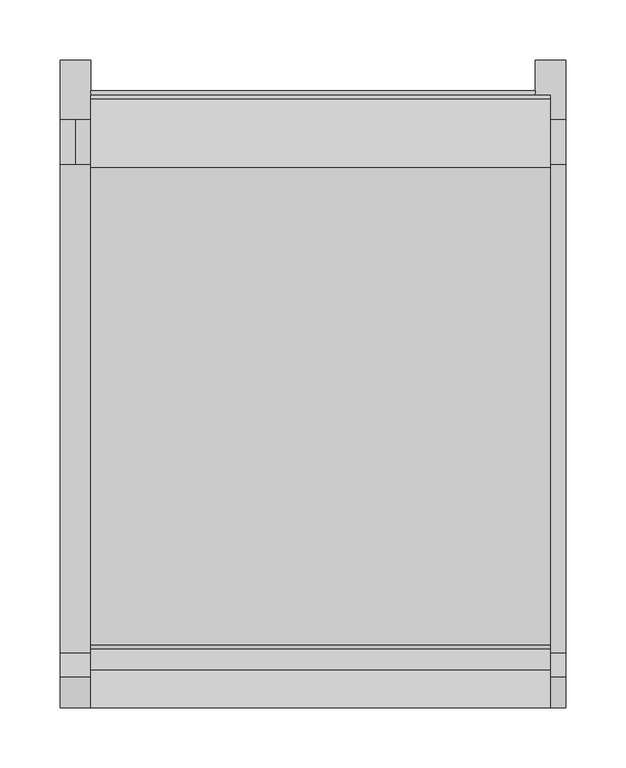
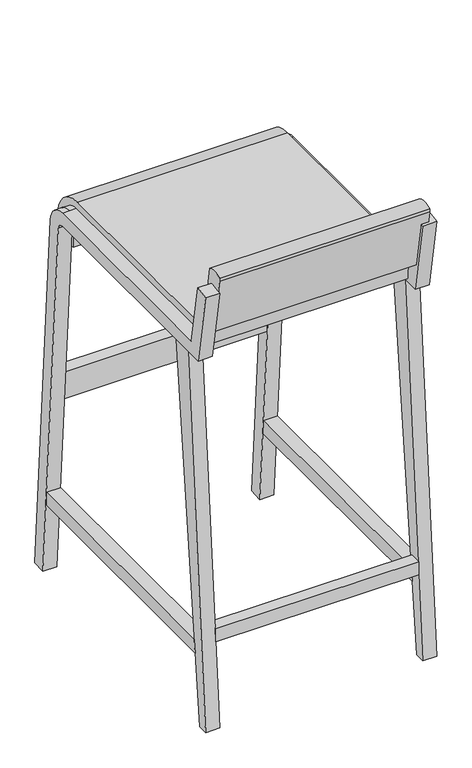
"""IFC4 building model written with IfcOpenShell, lengths in millimetres: furniture geometry, Bar_Stool_6722[1] : Bar_Stool_6722[1]."""

import ifcopenshell
import ifcopenshell.guid

model = None  # the IFC model being written
_history = None  # IfcOwnerHistory: only IFC2X3 demands one
_inside = {}  # id of a spatial element -> (the spatial element, [elements in it])
_under = {}  # id of a project, library or spatial element -> (it, [spatial elements below it])
_declared = {}  # id of a project -> (the project, [libraries it declares])
_typed = {}  # id of a type object -> (the type object, [elements of that type])
_made_of = {}  # id of a material, layer set ... -> (it, [elements and type objects made of it])


def new_model(schema):
    """Start an empty IFC model of exactly this schema.

    Asked for "IFC4X3", IfcOpenShell would pick the latest addendum, in which some entities
    have other attributes; the version numbers below select the first issue.
    IFC2X3 requires an IfcOwnerHistory on every rooted entity: one is made here for all.
    """
    global model, _history
    if schema == "IFC4X3":
        model = ifcopenshell.file(schema_version=(4, 3, 0, 0))
    else:
        model = ifcopenshell.file(schema=schema)
    _inside.clear()
    _under.clear()
    _declared.clear()
    _typed.clear()
    _made_of.clear()
    _history = None
    if model.schema == "IFC2X3":
        org = make("IfcOrganization", Name="unknown")
        user = make(
            "IfcPersonAndOrganization",
            ThePerson=make("IfcPerson", FamilyName="unknown"),
            TheOrganization=org,
        )
        app = make(
            "IfcApplication",
            ApplicationDeveloper=org,
            Version="unknown",
            ApplicationFullName="unknown",
            ApplicationIdentifier="unknown",
        )
        _history = make(
            "IfcOwnerHistory",
            OwningUser=user,
            OwningApplication=app,
            ChangeAction="ADDED",
            CreationDate=0,
        )
    return model


def make(cls, **values):
    """One entity of the class cls with the attributes given. An attribute that is None is left unset."""
    return model.create_entity(
        cls, **{name: value for name, value in values.items() if value is not None}
    )


def rooted(cls, **values):
    """An entity with a GlobalId (a new one), such as an element, a storey or a relation."""
    return make(cls, GlobalId=ifcopenshell.guid.new(), OwnerHistory=_history, **values)


def si_unit(unit_type, name, prefix=None):
    """IfcSIUnit, for example si_unit("LENGTHUNIT", "METRE", prefix="MILLI")."""
    return make("IfcSIUnit", UnitType=unit_type, Prefix=prefix, Name=name)


def assignment(units):
    """IfcUnitAssignment: the units of a project."""
    return None if units is None else make("IfcUnitAssignment", Units=units)


def point(xyz):
    """IfcCartesianPoint."""
    return None if xyz is None else make("IfcCartesianPoint", Coordinates=xyz)


def direction(xyz):
    """IfcDirection."""
    return None if xyz is None else make("IfcDirection", DirectionRatios=xyz)


def frame(location, z_axis=None, x_axis=None):
    """IfcAxis2Placement3D, a coordinate frame: its origin and axes. An axis left out is left unset."""
    return make(
        "IfcAxis2Placement3D",
        Location=point(location),
        Axis=direction(z_axis),
        RefDirection=direction(x_axis),
    )


def frame_2d(location, x_axis=None):
    """IfcAxis2Placement2D, a coordinate frame in the plane: its origin and x axis."""
    return make(
        "IfcAxis2Placement2D", Location=point(location), RefDirection=direction(x_axis)
    )


def origin():
    """The frame at (0, 0, 0) with its axes left unset."""
    return frame((0.0, 0.0, 0.0))


def place(relative_to, where):
    """IfcLocalPlacement: puts the frame where relative to a parent placement (None: the world)."""
    return make(
        "IfcLocalPlacement", PlacementRelTo=relative_to, RelativePlacement=where
    )


def context(
    kind, dimensions, precision=None, world=None, true_north=None, identifier=None
):
    """IfcGeometricRepresentationContext, for example the 3D "Model" context."""
    return make(
        "IfcGeometricRepresentationContext",
        ContextIdentifier=identifier,
        ContextType=kind,
        CoordinateSpaceDimension=dimensions,
        Precision=precision,
        WorldCoordinateSystem=world,
        TrueNorth=true_north,
    )


def project(units=None, contexts=None):
    """IfcProject with its units and contexts."""
    return rooted(
        "IfcProject",
        Name="project",
        RepresentationContexts=contexts,
        UnitsInContext=assignment(units),
    )


def spatial(cls, under=None, at=None, **own):
    """A site, building, storey or space (cls), placed at a placement, below another one or the project."""
    s = rooted(cls, ObjectPlacement=at, **own)
    if under is not None:
        _under.setdefault(under.id(), (under, []))[1].append(s)
    return s


def polyline(points):
    """IfcPolyline through the points."""
    return make("IfcPolyline", Points=[point(p) for p in points])


def circle_curve(where, radius):
    """IfcCircle in the frame where."""
    return make("IfcCircle", Position=where, Radius=radius)


def trimmed(basis, trim1, trim2, sense, master):
    """IfcTrimmedCurve: the piece of a basis curve between two trims."""
    return make(
        "IfcTrimmedCurve",
        BasisCurve=basis,
        Trim1=trim1,
        Trim2=trim2,
        SenseAgreement=sense,
        MasterRepresentation=master,
    )


def segment(curve, same_sense, transition):
    """IfcCompositeCurveSegment."""
    return make(
        "IfcCompositeCurveSegment",
        Transition=transition,
        SameSense=same_sense,
        ParentCurve=curve,
    )


def composite_curve(segments, self_intersect=None):
    """IfcCompositeCurve: segments joined end to end."""
    return make("IfcCompositeCurve", Segments=segments, SelfIntersect=self_intersect)


def outline(outer, holes=None, kind="AREA"):
    """IfcArbitraryClosedProfileDef: a profile drawn as a closed curve; with holes, ...WithVoids."""
    if holes is None:
        return make("IfcArbitraryClosedProfileDef", ProfileType=kind, OuterCurve=outer)
    return make(
        "IfcArbitraryProfileDefWithVoids",
        ProfileType=kind,
        OuterCurve=outer,
        InnerCurves=holes,
    )


def extrude(swept, where, along, depth):
    """IfcExtrudedAreaSolid: the profile swept, set in the frame where, extruded along a direction by depth."""
    return make(
        "IfcExtrudedAreaSolid",
        SweptArea=swept,
        Position=where,
        ExtrudedDirection=direction(along),
        Depth=depth,
    )


def shape(context_of_items, identifier, shape_type, items):
    """IfcShapeRepresentation: the items that make up one representation, for example the "Body"."""
    return make(
        "IfcShapeRepresentation",
        ContextOfItems=context_of_items,
        RepresentationIdentifier=identifier,
        RepresentationType=shape_type,
        Items=items,
    )


def source(mapping_origin, context_of_items, identifier, shape_type, items):
    """IfcRepresentationMap: a shape defined once, which mapped items show again and again."""
    return make(
        "IfcRepresentationMap",
        MappingOrigin=mapping_origin,
        MappedRepresentation=shape(context_of_items, identifier, shape_type, items),
    )


def transform(
    local_origin,
    x_axis=None,
    y_axis=None,
    z_axis=None,
    scale=None,
    scale2=None,
    scale3=None,
    uniform=True,
):
    """IfcCartesianTransformationOperator3D, or its non-uniform kind. x_axis, y_axis, z_axis: its Axis1, 2, 3."""
    if uniform:
        return make(
            "IfcCartesianTransformationOperator3D",
            Axis1=direction(x_axis),
            Axis2=direction(y_axis),
            LocalOrigin=point(local_origin),
            Scale=scale,
            Axis3=direction(z_axis),
        )
    return make(
        "IfcCartesianTransformationOperator3DnonUniform",
        Axis1=direction(x_axis),
        Axis2=direction(y_axis),
        LocalOrigin=point(local_origin),
        Scale=scale,
        Axis3=direction(z_axis),
        Scale2=scale2,
        Scale3=scale3,
    )


def mapped(mapping_source, mapping_target):
    """IfcMappedItem: shows the shape of a source again, moved by a transform."""
    return make(
        "IfcMappedItem", MappingSource=mapping_source, MappingTarget=mapping_target
    )


def made_of(thing, what):
    """Note that an element or type object is made of a material, layer set ...; save() writes the relation."""
    if what is not None:
        _made_of.setdefault(what.id(), (what, []))[1].append(thing)
    return thing


def element(
    cls,
    number,
    at=None,
    inside=None,
    cuts=None,
    type_object=None,
    material=None,
    context=None,
    identifier="Body",
    shape_type=None,
    held_by="IfcProductDefinitionShape",
    body=None,
    shapes=None,
    **own,
):
    """One element of the class cls, such as IfcWall. Its Tag is "e" and its number.

    at: its placement. inside: the storey or other place that contains it. cuts: it is an
    opening in that element (IfcRelVoidsElement). A single representation is given by context,
    identifier, shape_type and body (its items); several are given by shapes. held_by: the class
    of the entity that holds the representations. save() writes the other relations.
    """
    e = rooted(cls, Tag="e%d" % number, ObjectPlacement=at, **own)
    if body is not None:
        shapes = [shape(context, identifier, shape_type, body)]
    if shapes is not None:
        e.Representation = make(held_by, Representations=shapes)
    if inside is not None:
        _inside.setdefault(inside.id(), (inside, []))[1].append(e)
    if cuts is not None:
        rooted(
            "IfcRelVoidsElement", RelatingBuildingElement=cuts, RelatedOpeningElement=e
        )
    if type_object is not None:
        _typed.setdefault(type_object.id(), (type_object, []))[1].append(e)
    return made_of(e, material)


def aggregate(whole, parts):
    """IfcRelAggregates: a whole, such as a stair, and the parts it consists of."""
    return rooted("IfcRelAggregates", RelatingObject=whole, RelatedObjects=parts)


def save(model, path):
    """Write the relations noted so far, then the file.

    IfcRelAggregates (storeys below a building ...), IfcRelContainedInSpatialStructure (elements
    in a storey), IfcRelDefinesByType, IfcRelAssociatesMaterial and IfcRelDeclares: one each for
    every whole, place, type object, material and project.
    """
    for whole, parts in _under.values():
        aggregate(whole, parts)
    for where, things in _inside.values():
        rooted(
            "IfcRelContainedInSpatialStructure",
            RelatedElements=things,
            RelatingStructure=where,
        )
    for kind, things in _typed.values():
        rooted("IfcRelDefinesByType", RelatedObjects=things, RelatingType=kind)
    for what, things in _made_of.values():
        rooted("IfcRelAssociatesMaterial", RelatedObjects=things, RelatingMaterial=what)
    for by, libraries in _declared.values():
        rooted("IfcRelDeclares", RelatingContext=by, RelatedDefinitions=libraries)
    model.write(path)


def plane_surface(at):
    """IfcPlane: the flat surface through the origin of the frame at, square to its z axis."""
    return make("IfcPlane", Position=at)


def cylinder_surface(at, radius):
    """IfcCylindricalSurface: all points at the distance radius from the z axis of the frame at."""
    return make("IfcCylindricalSurface", Position=at, Radius=radius)


def revolved_surface(curve, axis_point, axis_direction):
    """IfcSurfaceOfRevolution: the curve turned about the line through axis_point along axis_direction."""
    return make(
        "IfcSurfaceOfRevolution",
        SweptCurve=make("IfcArbitraryOpenProfileDef", ProfileType="CURVE", Curve=curve),
        AxisPosition=make("IfcAxis1Placement", Location=point(axis_point), Axis=direction(axis_direction)),
    )


def advanced_brep(points, edges, surfaces, faces):
    """IfcAdvancedBrep: a solid bounded by faces that lie on surfaces and meet in shared edges.

    An edge is (start, end): straight between two places in points (the first is 0);
    or (start, end, curve); or (start, end, curve, False) where it runs against its curve.
    A face is (place in surfaces, loops), or (place, loops, False) where it looks against
    its surface's normal. A loop lists edges by number (the first is 1), with a minus sign
    where the edge is run from its end to its start. The first loop is the outer one.
    """
    corners = [point(p) for p in points]
    vertices = [make("IfcVertexPoint", VertexGeometry=c) for c in corners]
    made = []
    for start, end, *more in edges:
        made.append(
            make(
                "IfcEdgeCurve",
                EdgeStart=vertices[start],
                EdgeEnd=vertices[end],
                EdgeGeometry=more[0] if more else make("IfcPolyline", Points=[corners[start], corners[end]]),
                SameSense=more[1] if len(more) > 1 else True,
            )
        )
    hull = []
    for where, loops, *sense in faces:
        bounds = []
        for j, loop in enumerate(loops):
            ring = [make("IfcOrientedEdge", EdgeElement=made[abs(k) - 1], Orientation=k > 0) for k in loop]
            bounds.append(
                make(
                    "IfcFaceOuterBound" if j == 0 else "IfcFaceBound",
                    Bound=make("IfcEdgeLoop", EdgeList=ring),
                    Orientation=True,
                )
            )
        hull.append(make("IfcAdvancedFace", Bounds=bounds, FaceSurface=surfaces[where], SameSense=sense[0] if sense else True))
    return make("IfcAdvancedBrep", Outer=make("IfcClosedShell", CfsFaces=hull))


def furniture_d221970b(model_context):
    return source(origin(), model_context, "Body", "SolidModel", [
        advanced_brep(
        [(419.1, 25.0141169, 838.4759165), (393.7, 25.0141169, 838.4759165), (393.7, 0.0, 834.0652528), (419.1, 0.0, 834.0652528), (419.1, 45.2169423, 723.9), (393.7, 45.2169423, 723.9), (393.7, 450.0350637, 723.9), (393.7, 488.0397183, 688.4937383), (393.7, 536.7759384, 0.8979128), (393.7, 511.439502, -0.8979128), (393.7, 462.7032819, 686.6979128), (393.7, 450.0350637, 698.5), (393.7, 23.9038117, 698.5), (419.1, 23.9038117, 698.5), (419.1, 450.0350637, 698.5), (419.1, 462.7032819, 686.6979128), (419.1, 511.439502, -0.8979128), (419.1, 536.7759384, 0.8979128), (419.1, 488.0397183, 688.4937383), (419.1, 450.0350637, 723.9), (406.4, 450.0350637, 723.9), (406.4, 488.0397183, 688.4937383)],
        [
            (0, 1),
            (1, 2),
            (2, 3),
            (3, 0),
            (0, 4),
            (4, 5),
            (5, 1),
            (5, 6),
            (6, 7, circle_curve(frame((393.7, 450.0350637, 685.8), z_axis=(-1.0, 0.0, 0.0), x_axis=(0.0, 0.0, 1.0)), 38.1)),
            (7, 8),
            (8, 9),
            (9, 10),
            (10, 11, circle_curve(frame((393.7, 450.0350637, 685.8), z_axis=(1.0, 0.0, 0.0), x_axis=(0.0, 0.0, 1.0)), 12.7)),
            (11, 12),
            (12, 2),
            (12, 13),
            (13, 3),
            (13, 14),
            (14, 15, circle_curve(frame((419.1, 450.0350637, 685.8), z_axis=(-1.0, 0.0, 0.0), x_axis=(0.0, 0.0, 1.0)), 12.7)),
            (15, 16),
            (16, 17),
            (17, 18),
            (18, 19, circle_curve(frame((419.1, 450.0350637, 685.8), z_axis=(1.0, 0.0, 0.0), x_axis=(0.0, 0.0, 1.0)), 38.1)),
            (19, 4),
            (19, 20),
            (20, 6),
            (11, 14),
            (21, 20, circle_curve(frame((406.4, 450.0350637, 685.8), z_axis=(1.0, 0.0, 0.0), x_axis=(0.0, 0.0, 1.0)), 38.1)),
            (18, 21),
            (21, 7),
            (10, 15),
            (17, 8),
            (9, 16),
        ],
        [
            plane_surface(frame((406.4, 12.5070585, 836.2705846), z_axis=(0.0, -0.17364817766692853, 0.9848077530122085), x_axis=(1.0, 0.0, 0.0))),
            plane_surface(frame((406.4, 25.0141169, 838.4759165), z_axis=(0.0, 0.9848077530122085, 0.17364817766692814), x_axis=(0.0, 0.17364817766692814, -0.9848077530122085))),
            plane_surface(frame((393.7, 25.0141169, 838.4759165), z_axis=(-1.0, 0.0, 0.0), x_axis=(0.0, 0.17364817766692808, -0.9848077530122085))),
            plane_surface(frame((393.7, 0.0, 834.0652528), z_axis=(0.0, -0.9848077530122085, -0.17364817766692817), x_axis=(0.0, 0.17364817766692817, -0.9848077530122085))),
            plane_surface(frame((419.1, 0.0, 834.0652528), z_axis=(1.0000000000000002, 0.0, 0.0), x_axis=(0.0, 0.1736481776669284, -0.9848077530122085))),
            plane_surface(frame((406.4, 45.2169423, 723.9), z_axis=(0.0, 0.0, 1.0), x_axis=(0.0, 1.0, 0.0))),
            plane_surface(frame((393.7, 23.9038117, 698.5), z_axis=(0.0, 0.0, -1.0), x_axis=(0.0, 1.0, 0.0))),
            cylinder_surface(frame((406.4, 450.0350637, 685.8), z_axis=(-1.0, 0.0, 0.0), x_axis=(0.0, 0.0, 1.0)), 38.1),
            revolved_surface(polyline([(393.7, 450.0350637, 698.5), (419.1, 450.0350637, 698.5)]), (406.4, 450.0350637, 685.8), (-1.0, 0.0, 0.0)),
            plane_surface(frame((406.4, 488.0397183, 688.4937383), z_axis=(0.0, 0.9974974969901172, 0.07070179275273744), x_axis=(0.0, 0.07070179275273744, -0.9974974969901172))),
            plane_surface(frame((393.7, 462.7032819, 686.6979128), z_axis=(0.0, -0.9974974969901172, -0.07070179275273743), x_axis=(0.0, 0.07070179275273743, -0.9974974969901172))),
            plane_surface(frame((406.4, 524.1077202, 0.0), z_axis=(0.0, 0.07070179275273399, -0.9974974969901175), x_axis=(1.0, 0.0, 0.0))),
        ],
        [
            (0, [[1, 2, 3, 4]]),
            (1, [[5, 6, 7, -1]]),
            (2, [[-2, -7, 8, 9, 10, 11, 12, 13, 14, 15]]),
            (3, [[-3, -15, 16, 17]]),
            (4, [[-4, -17, 18, 19, 20, 21, 22, 23, 24, -5]]),
            (5, [[-6, -24, 25, 26, -8]]),
            (6, [[-16, -14, 27, -18]]),
            (7, [[28, -25, -23, 29]]),
            (7, [[-9, -26, -28, 30]]),
            (8, [[-19, -27, -13, 31]]),
            (9, [[-10, -30, -29, -22, 32]]),
            (10, [[-20, -31, -12, 33]]),
            (11, [[-32, -21, -33, -11]]),
        ],
    ),
        extrude(outline(composite_curve([segment(polyline([(48.4096386, 756.5644068), (44.0710693, 752.2258375), (19.1416957, 748.2774126), (0.0, 856.8353632), (0.0, 863.1853632)]), True, "CONTINUOUS"), segment(trimmed(circle_curve(frame_2d((15.7612691, 828.3540875)), 38.2313401), [point((0.0, 863.1853632))], [point((31.5225381, 863.1853632))], False, "CARTESIAN"), True, "CONTINUOUS"), segment(polyline([(31.5225381, 863.1853632), (48.4096386, 756.5644068)]), True, "CONTINUOUS")], self_intersect=False)), frame((25.4, 0.0, 0.0), z_axis=(1.0, 0.0, 0.0), x_axis=(0.0, 1.0, 0.0)), (0.0, 0.0, 1.0), 381.0),
        extrude(outline(composite_curve([segment(polyline([(51.6744261, 737.5144068), (447.8968201, 737.5144068)]), True, "CONTINUOUS"), segment(trimmed(circle_curve(frame_2d((447.8968201, 676.6245275)), 60.8898793), [point((447.8968201, 737.5144068))], [point((505.1145904, 697.4500928))], False, "CARTESIAN"), True, "CONTINUOUS"), segment(trimmed(circle_curve(frame_2d((460.5585493, 681.23302)), 47.4155486), [point((505.1145904, 697.4500928))], [point((484.2663236, 640.1699505))], False, "CARTESIAN"), True, "CONTINUOUS"), segment(polyline([(484.2663236, 640.1699505), (460.5585493, 643.13302), (460.5585493, 681.23302), (452.817441, 704.85), (46.417441, 704.85), (43.9498561, 733.0546243), (51.6744261, 737.5144068)]), True, "CONTINUOUS")], self_intersect=False)), frame((25.4, 0.0, 0.0), z_axis=(1.0, 0.0, 0.0), x_axis=(0.0, 1.0, 0.0)), (0.0, 0.0, 1.0), 381.0),
        extrude(outline(polyline([(393.7, 11.6871233), (25.4, 11.6871233), (25.4, 33.1441574), (393.7, 33.1441574), (393.7, 11.6871233)])), frame((0.0, 0.0, 157.9619127), z_axis=(0.0, 0.0, 1.0), x_axis=(1.0, 0.0, 0.0)), (0.0, 0.0, 1.0), 25.4),
        extrude(outline(polyline([(393.7, 488.2695397), (25.4, 488.2695397), (25.4, 511.439502), (393.7, 511.439502), (393.7, 488.2695397)])), frame((0.0, 0.0, 335.7619127), z_axis=(0.0, 0.0, 1.0), x_axis=(1.0, 0.0, 0.0)), (0.0, 0.0, 1.0), 50.8),
        extrude(outline(polyline([(500.1796497, 157.9619127), (500.1796497, 132.5619127), (32.9828185, 132.5619127), (35.652466, 157.9619127), (500.1796497, 157.9619127)])), frame((393.7, 0.0, 0.0), z_axis=(1.0, 0.0, 0.0), x_axis=(0.0, 1.0, 0.0)), (0.0, 0.0, 1.0), 25.4),
        extrude(outline(polyline([(500.1796497, 157.9619127), (500.1796497, 132.5619127), (32.9828185, 132.5619127), (35.652466, 157.9619127), (500.1796497, 157.9619127)])), frame((0.0, 0.0, 0.0), z_axis=(1.0, 0.0, 0.0), x_axis=(0.0, 1.0, 0.0)), (0.0, 0.0, 1.0), 25.4),
        extrude(outline(polyline([(0.0, 0.0), (55.3031462, 698.5), (92.4653083, 698.5), (19.05, 0.0), (0.0, 0.0)])), frame((393.7, 0.0, 0.0), z_axis=(1.0, 0.0, 0.0), x_axis=(0.0, 1.0, 0.0)), (0.0, 0.0, 1.0), 25.4),
        advanced_brep(
        [(25.4, 25.0141169, 838.4759165), (0.0, 25.0141169, 838.4759165), (0.0, 0.0, 834.0652528), (25.4, 0.0, 834.0652528), (25.4, 45.2169423, 723.9), (0.0, 45.2169423, 723.9), (0.0, 450.0350637, 723.9), (0.0, 488.0397183, 688.4937383), (0.0, 536.7759384, 0.8979128), (0.0, 511.439502, -0.8979128), (0.0, 462.7032819, 686.6979128), (0.0, 450.0350637, 698.5), (0.0, 23.9038117, 698.5), (25.4, 23.9038117, 698.5), (25.4, 450.0350637, 698.5), (25.4, 462.7032819, 686.6979128), (25.4, 511.439502, -0.8979128), (25.4, 536.7759384, 0.8979128), (25.4, 488.0397183, 688.4937383), (25.4, 450.0350637, 723.9), (12.7, 450.0350637, 723.9), (12.7, 488.0397183, 688.4937383)],
        [
            (0, 1),
            (1, 2),
            (2, 3),
            (3, 0),
            (0, 4),
            (4, 5),
            (5, 1),
            (5, 6),
            (6, 7, circle_curve(frame((0.0, 450.0350637, 685.8), z_axis=(-1.0, 0.0, 0.0), x_axis=(0.0, 0.0, 1.0)), 38.1)),
            (7, 8),
            (8, 9),
            (9, 10),
            (10, 11, circle_curve(frame((0.0, 450.0350637, 685.8), z_axis=(1.0, 0.0, 0.0), x_axis=(0.0, 0.0, 1.0)), 12.7)),
            (11, 12),
            (12, 2),
            (12, 13),
            (13, 3),
            (13, 14),
            (14, 15, circle_curve(frame((25.4, 450.0350637, 685.8), z_axis=(-1.0, 0.0, 0.0), x_axis=(0.0, 0.0, 1.0)), 12.7)),
            (15, 16),
            (16, 17),
            (17, 18),
            (18, 19, circle_curve(frame((25.4, 450.0350637, 685.8), z_axis=(1.0, 0.0, 0.0), x_axis=(0.0, 0.0, 1.0)), 38.1)),
            (19, 4),
            (19, 20),
            (20, 6),
            (11, 14),
            (7, 21),
            (21, 18),
            (17, 8),
            (15, 10),
            (9, 16),
            (21, 20, circle_curve(frame((12.7, 450.0350637, 685.8), z_axis=(1.0, 0.0, 0.0), x_axis=(0.0, 0.0, 1.0)), 38.1)),
        ],
        [
            plane_surface(frame((12.7, 12.5070585, 836.2705846), z_axis=(0.0, -0.17364817766692853, 0.9848077530122085), x_axis=(1.0, 0.0, 0.0))),
            plane_surface(frame((12.7, 25.0141169, 838.4759165), z_axis=(0.0, 0.9848077530122085, 0.173648177666928), x_axis=(0.0, 0.173648177666928, -0.9848077530122085))),
            plane_surface(frame((0.0, 25.0141169, 838.4759165), z_axis=(-1.0, 0.0, 0.0), x_axis=(0.0, 0.17364817766692875, -0.9848077530122084))),
            plane_surface(frame((0.0, 0.0, 834.0652528), z_axis=(0.0, -0.9848077530122084, -0.17364817766692883), x_axis=(0.0, 0.17364817766692883, -0.9848077530122084))),
            plane_surface(frame((25.4, 0.0, 834.0652528), z_axis=(1.0000000000000002, 0.0, 0.0), x_axis=(0.0, 0.1736481776669284, -0.9848077530122085))),
            plane_surface(frame((12.7, 45.2169423, 723.9), z_axis=(0.0, 0.0, 1.0), x_axis=(0.0, 1.0, 0.0))),
            plane_surface(frame((0.0, 23.9038117, 698.5), z_axis=(0.0, 0.0, -1.0), x_axis=(0.0, 1.0, 0.0))),
            plane_surface(frame((12.7, 488.0397183, 688.4937383), z_axis=(0.0, 0.9974974969901172, 0.07070179275273744), x_axis=(0.0, 0.07070179275273744, -0.9974974969901172))),
            plane_surface(frame((0.0, 462.7032819, 686.6979128), z_axis=(0.0, -0.9974974969901172, -0.07070179275273743), x_axis=(0.0, 0.07070179275273743, -0.9974974969901172))),
            plane_surface(frame((12.7, 524.1077202, 0.0), z_axis=(0.0, 0.07070179275273399, -0.9974974969901175), x_axis=(1.0, 0.0, 0.0))),
            cylinder_surface(frame((12.7, 450.0350637, 685.8), z_axis=(-1.0, 0.0, 0.0), x_axis=(0.0, 0.0, 1.0)), 38.1),
            revolved_surface(polyline([(0.0, 450.0350637, 698.5), (25.4, 450.0350637, 698.5)]), (12.7, 450.0350637, 685.8), (-1.0, 0.0, 0.0)),
        ],
        [
            (0, [[1, 2, 3, 4]]),
            (1, [[5, 6, 7, -1]]),
            (2, [[-2, -7, 8, 9, 10, 11, 12, 13, 14, 15]]),
            (3, [[-3, -15, 16, 17]]),
            (4, [[-4, -17, 18, 19, 20, 21, 22, 23, 24, -5]]),
            (5, [[-6, -24, 25, 26, -8]]),
            (6, [[-16, -14, 27, -18]]),
            (7, [[-10, 28, 29, -22, 30]]),
            (8, [[-20, 31, -12, 32]]),
            (9, [[-30, -21, -32, -11]]),
            (10, [[33, -25, -23, -29]]),
            (10, [[-9, -26, -33, -28]]),
            (11, [[-19, -27, -13, -31]]),
        ],
    ),
        extrude(outline(polyline([(0.0, 0.0), (55.3031462, 698.5), (92.4653083, 698.5), (19.05, 0.0), (0.0, 0.0)])), frame((0.0, 0.0, 0.0), z_axis=(1.0, 0.0, 0.0), x_axis=(0.0, 1.0, 0.0)), (0.0, 0.0, 1.0), 25.4),
    ])


if __name__ == "__main__":
    model = new_model("IFC4")
    model_context = context("Model", 3, world=origin())
    ifc_project = project(units=[si_unit("LENGTHUNIT", "METRE", prefix="MILLI")], contexts=[model_context])
    site = spatial("IfcSite", under=ifc_project)
    building = spatial("IfcBuilding", under=site)
    placement = place(None, origin())
    furniture_shape = furniture_d221970b(model_context)
    element("IfcFurniture", 1, ObjectType="Bar_Stool_6722[1] : Bar_Stool_6722[1]", at=placement, inside=building, context=model_context, shape_type="MappedRepresentation", body=[
        mapped(furniture_shape, transform((0.0, 0.0, 0.0), x_axis=(1.0, 0.0, 0.0), y_axis=(0.0, 1.0, 0.0), z_axis=(0.0, 0.0, 1.0))),
    ])
    save(model, "model.ifc")

# Revit data of these elements
# Type "Bar_Stool_6722[1] : Bar_Stool_6722[1]"
#   Seat = fab
#   Chair Legs = MET
# Element 1 (IfcFurniture, "Bar_Stool_6722[1] : Bar_Stool_6722[1]")
#   Materials on its faces: "MET", "fab"
# Materials
#   "fab": class "Leather", colour RGB 99 104 100, transparency 0
#   "MET": class "Metal", colour RGB 189 187 185, transparency 0
